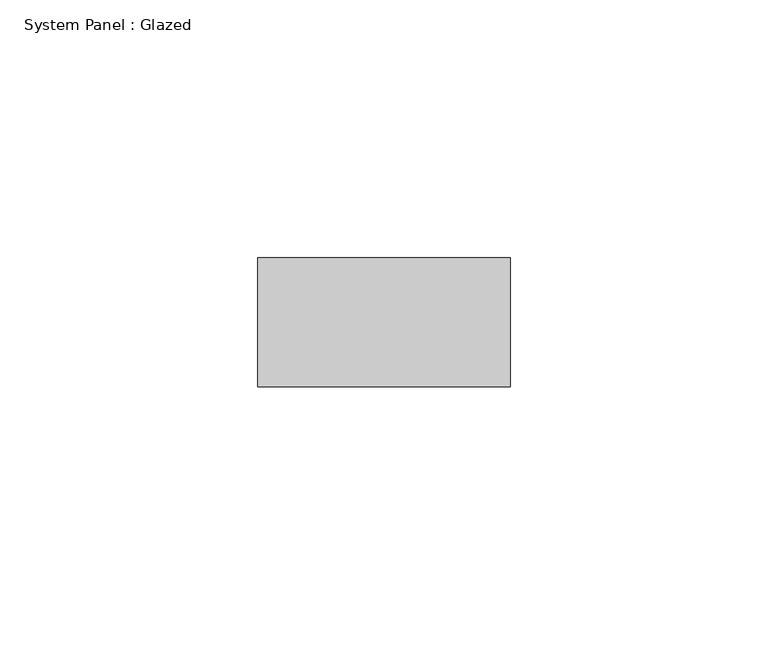
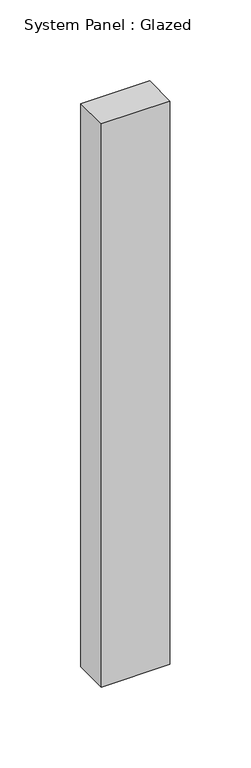
"""IFC4 building model written with IfcOpenShell, lengths in millimetres: plate geometry, System Panel : Glazed."""

import ifcopenshell
import ifcopenshell.guid

model = None  # the IFC model being written
_history = None  # IfcOwnerHistory: only IFC2X3 demands one
_inside = {}  # id of a spatial element -> (the spatial element, [elements in it])
_under = {}  # id of a project, library or spatial element -> (it, [spatial elements below it])
_declared = {}  # id of a project -> (the project, [libraries it declares])
_typed = {}  # id of a type object -> (the type object, [elements of that type])
_made_of = {}  # id of a material, layer set ... -> (it, [elements and type objects made of it])


def new_model(schema):
    """Start an empty IFC model of exactly this schema.

    Asked for "IFC4X3", IfcOpenShell would pick the latest addendum, in which some entities
    have other attributes; the version numbers below select the first issue.
    IFC2X3 requires an IfcOwnerHistory on every rooted entity: one is made here for all.
    """
    global model, _history
    if schema == "IFC4X3":
        model = ifcopenshell.file(schema_version=(4, 3, 0, 0))
    else:
        model = ifcopenshell.file(schema=schema)
    _inside.clear()
    _under.clear()
    _declared.clear()
    _typed.clear()
    _made_of.clear()
    _history = None
    if model.schema == "IFC2X3":
        org = make("IfcOrganization", Name="unknown")
        user = make(
            "IfcPersonAndOrganization",
            ThePerson=make("IfcPerson", FamilyName="unknown"),
            TheOrganization=org,
        )
        app = make(
            "IfcApplication",
            ApplicationDeveloper=org,
            Version="unknown",
            ApplicationFullName="unknown",
            ApplicationIdentifier="unknown",
        )
        _history = make(
            "IfcOwnerHistory",
            OwningUser=user,
            OwningApplication=app,
            ChangeAction="ADDED",
            CreationDate=0,
        )
    return model


def make(cls, **values):
    """One entity of the class cls with the attributes given. An attribute that is None is left unset."""
    return model.create_entity(
        cls, **{name: value for name, value in values.items() if value is not None}
    )


def rooted(cls, **values):
    """An entity with a GlobalId (a new one), such as an element, a storey or a relation."""
    return make(cls, GlobalId=ifcopenshell.guid.new(), OwnerHistory=_history, **values)


def si_unit(unit_type, name, prefix=None):
    """IfcSIUnit, for example si_unit("LENGTHUNIT", "METRE", prefix="MILLI")."""
    return make("IfcSIUnit", UnitType=unit_type, Prefix=prefix, Name=name)


def assignment(units):
    """IfcUnitAssignment: the units of a project."""
    return None if units is None else make("IfcUnitAssignment", Units=units)


def point(xyz):
    """IfcCartesianPoint."""
    return None if xyz is None else make("IfcCartesianPoint", Coordinates=xyz)


def direction(xyz):
    """IfcDirection."""
    return None if xyz is None else make("IfcDirection", DirectionRatios=xyz)


def frame(location, z_axis=None, x_axis=None):
    """IfcAxis2Placement3D, a coordinate frame: its origin and axes. An axis left out is left unset."""
    return make(
        "IfcAxis2Placement3D",
        Location=point(location),
        Axis=direction(z_axis),
        RefDirection=direction(x_axis),
    )


def origin():
    """The frame at (0, 0, 0) with its axes left unset."""
    return frame((0.0, 0.0, 0.0))


def origin_with_axes():
    """The frame at (0, 0, 0) with the z axis (0, 0, 1) and the x axis (1, 0, 0) written out."""
    return frame((0.0, 0.0, 0.0), z_axis=(0.0, 0.0, 1.0), x_axis=(1.0, 0.0, 0.0))


def place(relative_to, where):
    """IfcLocalPlacement: puts the frame where relative to a parent placement (None: the world)."""
    return make(
        "IfcLocalPlacement", PlacementRelTo=relative_to, RelativePlacement=where
    )


def context(
    kind, dimensions, precision=None, world=None, true_north=None, identifier=None
):
    """IfcGeometricRepresentationContext, for example the 3D "Model" context."""
    return make(
        "IfcGeometricRepresentationContext",
        ContextIdentifier=identifier,
        ContextType=kind,
        CoordinateSpaceDimension=dimensions,
        Precision=precision,
        WorldCoordinateSystem=world,
        TrueNorth=true_north,
    )


def project(units=None, contexts=None):
    """IfcProject with its units and contexts."""
    return rooted(
        "IfcProject",
        Name="project",
        RepresentationContexts=contexts,
        UnitsInContext=assignment(units),
    )


def spatial(cls, under=None, at=None, **own):
    """A site, building, storey or space (cls), placed at a placement, below another one or the project."""
    s = rooted(cls, ObjectPlacement=at, **own)
    if under is not None:
        _under.setdefault(under.id(), (under, []))[1].append(s)
    return s


def polyline(points):
    """IfcPolyline through the points."""
    return make("IfcPolyline", Points=[point(p) for p in points])


def outline(outer, holes=None, kind="AREA"):
    """IfcArbitraryClosedProfileDef: a profile drawn as a closed curve; with holes, ...WithVoids."""
    if holes is None:
        return make("IfcArbitraryClosedProfileDef", ProfileType=kind, OuterCurve=outer)
    return make(
        "IfcArbitraryProfileDefWithVoids",
        ProfileType=kind,
        OuterCurve=outer,
        InnerCurves=holes,
    )


def extrude(swept, where, along, depth):
    """IfcExtrudedAreaSolid: the profile swept, set in the frame where, extruded along a direction by depth."""
    return make(
        "IfcExtrudedAreaSolid",
        SweptArea=swept,
        Position=where,
        ExtrudedDirection=direction(along),
        Depth=depth,
    )


def shape(context_of_items, identifier, shape_type, items):
    """IfcShapeRepresentation: the items that make up one representation, for example the "Body"."""
    return make(
        "IfcShapeRepresentation",
        ContextOfItems=context_of_items,
        RepresentationIdentifier=identifier,
        RepresentationType=shape_type,
        Items=items,
    )


def source(mapping_origin, context_of_items, identifier, shape_type, items):
    """IfcRepresentationMap: a shape defined once, which mapped items show again and again."""
    return make(
        "IfcRepresentationMap",
        MappingOrigin=mapping_origin,
        MappedRepresentation=shape(context_of_items, identifier, shape_type, items),
    )


def transform(
    local_origin,
    x_axis=None,
    y_axis=None,
    z_axis=None,
    scale=None,
    scale2=None,
    scale3=None,
    uniform=True,
):
    """IfcCartesianTransformationOperator3D, or its non-uniform kind. x_axis, y_axis, z_axis: its Axis1, 2, 3."""
    if uniform:
        return make(
            "IfcCartesianTransformationOperator3D",
            Axis1=direction(x_axis),
            Axis2=direction(y_axis),
            LocalOrigin=point(local_origin),
            Scale=scale,
            Axis3=direction(z_axis),
        )
    return make(
        "IfcCartesianTransformationOperator3DnonUniform",
        Axis1=direction(x_axis),
        Axis2=direction(y_axis),
        LocalOrigin=point(local_origin),
        Scale=scale,
        Axis3=direction(z_axis),
        Scale2=scale2,
        Scale3=scale3,
    )


def mapped(mapping_source, mapping_target):
    """IfcMappedItem: shows the shape of a source again, moved by a transform."""
    return make(
        "IfcMappedItem", MappingSource=mapping_source, MappingTarget=mapping_target
    )


def made_of(thing, what):
    """Note that an element or type object is made of a material, layer set ...; save() writes the relation."""
    if what is not None:
        _made_of.setdefault(what.id(), (what, []))[1].append(thing)
    return thing


def element(
    cls,
    number,
    at=None,
    inside=None,
    cuts=None,
    type_object=None,
    material=None,
    context=None,
    identifier="Body",
    shape_type=None,
    held_by="IfcProductDefinitionShape",
    body=None,
    shapes=None,
    **own,
):
    """One element of the class cls, such as IfcWall. Its Tag is "e" and its number.

    at: its placement. inside: the storey or other place that contains it. cuts: it is an
    opening in that element (IfcRelVoidsElement). A single representation is given by context,
    identifier, shape_type and body (its items); several are given by shapes. held_by: the class
    of the entity that holds the representations. save() writes the other relations.
    """
    e = rooted(cls, Tag="e%d" % number, ObjectPlacement=at, **own)
    if body is not None:
        shapes = [shape(context, identifier, shape_type, body)]
    if shapes is not None:
        e.Representation = make(held_by, Representations=shapes)
    if inside is not None:
        _inside.setdefault(inside.id(), (inside, []))[1].append(e)
    if cuts is not None:
        rooted(
            "IfcRelVoidsElement", RelatingBuildingElement=cuts, RelatedOpeningElement=e
        )
    if type_object is not None:
        _typed.setdefault(type_object.id(), (type_object, []))[1].append(e)
    return made_of(e, material)


def aggregate(whole, parts):
    """IfcRelAggregates: a whole, such as a stair, and the parts it consists of."""
    return rooted("IfcRelAggregates", RelatingObject=whole, RelatedObjects=parts)


def save(model, path):
    """Write the relations noted so far, then the file.

    IfcRelAggregates (storeys below a building ...), IfcRelContainedInSpatialStructure (elements
    in a storey), IfcRelDefinesByType, IfcRelAssociatesMaterial and IfcRelDeclares: one each for
    every whole, place, type object, material and project.
    """
    for whole, parts in _under.values():
        aggregate(whole, parts)
    for where, things in _inside.values():
        rooted(
            "IfcRelContainedInSpatialStructure",
            RelatedElements=things,
            RelatingStructure=where,
        )
    for kind, things in _typed.values():
        rooted("IfcRelDefinesByType", RelatedObjects=things, RelatingType=kind)
    for what, things in _made_of.values():
        rooted("IfcRelAssociatesMaterial", RelatedObjects=things, RelatingMaterial=what)
    for by, libraries in _declared.values():
        rooted("IfcRelDeclares", RelatingContext=by, RelatedDefinitions=libraries)
    model.write(path)


def system_panel_glazed_0535c902(model_context):
    return source(origin(), model_context, "Body", "SweptSolid", [
        extrude(outline(polyline([(24.5092572, -49.5), (-24.5092572, -49.5), (-24.5092572, -24.5), (24.5092572, -24.5), (24.5092572, -49.5)])), origin_with_axes(), (0.0, 0.0, 1.0), 425.0),
    ])


if __name__ == "__main__":
    model = new_model("IFC4")
    model_context = context("Model", 3, world=origin())
    ifc_project = project(units=[si_unit("LENGTHUNIT", "METRE", prefix="MILLI")], contexts=[model_context])
    site = spatial("IfcSite", under=ifc_project)
    building = spatial("IfcBuilding", under=site)
    placement = place(None, origin())
    system_panel_glazed_shape = system_panel_glazed_0535c902(model_context)
    element("IfcPlate", 1, ObjectType="System Panel : Glazed", at=placement, inside=building, context=model_context, shape_type="MappedRepresentation", body=[
        mapped(system_panel_glazed_shape, transform((0.0, 0.0, 0.0), x_axis=(1.0, 0.0, 0.0), y_axis=(0.0, 1.0, 0.0), z_axis=(0.0, 0.0, 1.0))),
    ])
    save(model, "model.ifc")

# Revit data of these elements
# Type "System Panel : Glazed"
#   Keynote = "H11"
#   Construction Type Id = "GSP4R"
#   Analytic Construction = "1/8 in Pilkington single glazing"
#   Visual Light Transmittance = 0.9
#   Solar Heat Gain Coefficient = 0.86
#   Heat Transfer Coefficient (U) = 6.7069 W/(m²·K)
# Element 1 (IfcPlate, "System Panel : Glazed")
#   Materials on its faces: "Glass"
# Materials
#   "Glass": class "Glass", colour RGB 0 128 192, transparency 0.9, Description = "Soda Lime Glass", Cost = 0
